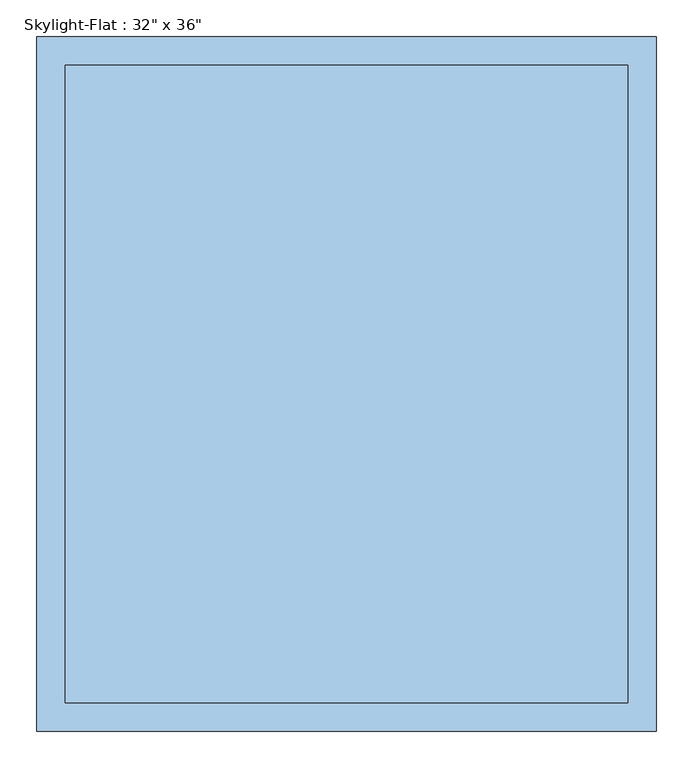
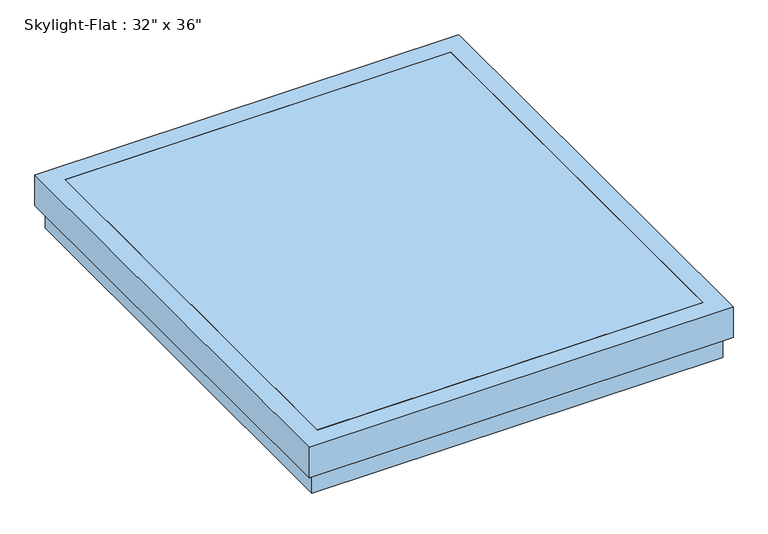
"""IFC4 building model written with IfcOpenShell, lengths in millimetres: window geometry."""

from ifc_helpers import new_model, si_unit, frame, origin, place, context, project, spatial, polyline, outline, extrude, faceted_brep, source, transform, mapped, element, save


def window_a8ca25b6(model_context):
    return source(origin(), model_context, "Body", "SolidModel", [
        extrude(outline(polyline([(381.0, 431.8), (381.0, -431.8), (-381.0, -431.8), (-381.0, 431.8), (381.0, 431.8)])), frame((0.0, 0.0, 3966.36875), z_axis=(0.0, 0.0, 1.0), x_axis=(1.0, 0.0, 0.0)), (0.0, 0.0, 1.0), 5.55625),
        faceted_brep([(419.1, 469.9, 3908.425), (419.1, 469.9, 3971.925), (419.1, -469.9, 3971.925), (419.1, -469.9, 3908.425), (406.4, 457.2, 3946.525), (406.4, 457.2, 3908.425), (406.4, -457.2, 3908.425), (406.4, -457.2, 3946.525), (381.0, 431.8, 3971.925), (381.0, 431.8, 3946.525), (381.0, -431.8, 3946.525), (381.0, -431.8, 3971.925), (-419.1, -469.9, 3971.925), (-419.1, -469.9, 3908.425), (-406.4, -457.2, 3908.425), (-406.4, -457.2, 3946.525), (-381.0, -431.8, 3946.525), (-381.0, -431.8, 3971.925), (-419.1, 469.9, 3971.925), (-419.1, 469.9, 3908.425), (-406.4, 457.2, 3908.425), (-406.4, 457.2, 3946.525), (-381.0, 431.8, 3946.525), (-381.0, 431.8, 3971.925)], [[[0, 1, 2, 3]], [[4, 5, 6, 7]], [[8, 9, 10, 11]], [[3, 2, 12, 13]], [[7, 6, 14, 15]], [[11, 10, 16, 17]], [[13, 12, 18, 19]], [[15, 14, 20, 21]], [[17, 16, 22, 23]], [[1, 18, 12, 2], [11, 17, 23, 8]], [[19, 18, 1, 0]], [[3, 13, 19, 0], [5, 20, 14, 6]], [[21, 20, 5, 4]], [[7, 15, 21, 4], [9, 22, 16, 10]], [[23, 22, 9, 8]]]),
        faceted_brep([(406.4, 457.2, 3863.975), (406.4, 457.2, 3946.525), (406.4, -457.2, 3946.525), (406.4, -457.2, 3863.975), (342.9, 393.7, 3921.125), (342.9, 393.7, 3863.975), (342.9, -393.7, 3863.975), (342.9, -393.7, 3921.125), (381.0, 431.8, 3946.525), (381.0, 431.8, 3921.125), (381.0, -431.8, 3921.125), (381.0, -431.8, 3946.525), (-406.4, -457.2, 3946.525), (-406.4, -457.2, 3863.975), (-342.9, -393.7, 3863.975), (-342.9, -393.7, 3921.125), (-381.0, -431.8, 3921.125), (-381.0, -431.8, 3946.525), (-406.4, 457.2, 3946.525), (-406.4, 457.2, 3863.975), (-342.9, 393.7, 3863.975), (-342.9, 393.7, 3921.125), (-381.0, 431.8, 3921.125), (-381.0, 431.8, 3946.525)], [[[0, 1, 2, 3]], [[4, 5, 6, 7]], [[8, 9, 10, 11]], [[3, 2, 12, 13]], [[7, 6, 14, 15]], [[11, 10, 16, 17]], [[13, 12, 18, 19]], [[15, 14, 20, 21]], [[17, 16, 22, 23]], [[19, 18, 1, 0]], [[3, 13, 19, 0], [5, 20, 14, 6]], [[21, 20, 5, 4]], [[9, 22, 16, 10], [7, 15, 21, 4]], [[23, 22, 9, 8]], [[1, 18, 12, 2], [11, 17, 23, 8]]]),
    ])


if __name__ == "__main__":
    model = new_model("IFC4")
    model_context = context("Model", 3, world=origin())
    ifc_project = project(units=[si_unit("LENGTHUNIT", "METRE", prefix="MILLI")], contexts=[model_context])
    site = spatial("IfcSite", under=ifc_project)
    building = spatial("IfcBuilding", under=site)
    placement = place(None, origin())
    window_shape = window_a8ca25b6(model_context)
    element("IfcWindow", 1, ObjectType="Skylight-Flat : 32\" x 36\"", at=placement, inside=building, context=model_context, shape_type="MappedRepresentation", body=[
        mapped(window_shape, transform((0.0, 0.0, 0.0), x_axis=(1.0, 0.0, 0.0), y_axis=(0.0, 1.0, 0.0), z_axis=(0.0, 0.0, 1.0))),
    ])
    save(model, "model.ifc")

# Revit data of these elements
# Type "Skylight-Flat : 32\" x 36\""
#   Type Mark = "25"
#   Fire Rating = "0.5h"
#   Assembly Code = "B2020100"
#   Analytic Construction = "Single-glazed windows - domestic"
#   Width = 2' - 8"
#   Visual Light Transmittance = 0.9
#   Thermal Resistance (R) = 0.9899 (h·ft²·°F)/BTU
#   Solar Heat Gain Coefficient = 0.86
#   Rough Width = 2' - 8 1/2"
#   Rough Height = 3' - 0 1/2"
#   Height = 3' - 0"
#   Heat Transfer Coefficient (U) = 1.0102 BTU/(h·ft²·°F)
#   Base Height = 0' - 3 1/4"
#   Glass Panel Material = Glass
#   Frame Material = Metal - Bronze, Light Brush
# Element 1 (IfcWindow, "Skylight-Flat : 32\" x 36\"")
#   Materials on its faces: "Metal - Bronze, Light Brush", "Glass"
# Materials
#   "Glass": class "Glass", colour RGB 0 128 192, transparency 0.75, Description = "Soda Lime Glass", Cost = 0
#   "Metal - Bronze, Light Brush": class "Metal", colour RGB 113 80 70, transparency 0
